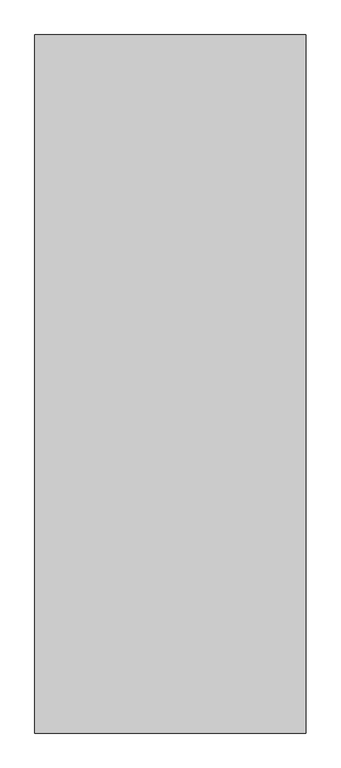
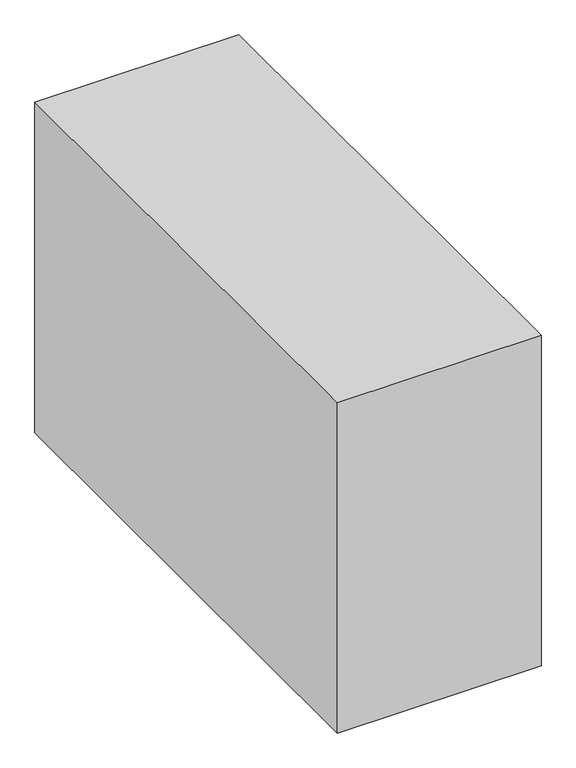
"""IFC4 building model written with IfcOpenShell, lengths in millimetres: proxy geometry, Space Planning Box_hec : Space Planning Box_hec."""

from ifc_helpers import new_model, si_unit, origin, origin_with_axes, place, context, project, spatial, polyline, outline, extrude, source, transform, mapped, element, save


def generic_models_c01b8d6f(model_context):
    return source(origin(), model_context, "Body", "SweptSolid", [
        extrude(outline(polyline([(1750.0, 4500.0), (1750.0, -4500.0), (-1750.0, -4500.0), (-1750.0, 4500.0), (1750.0, 4500.0)])), origin_with_axes(), (0.0, 0.0, 1.0), 6000.0),
    ])


if __name__ == "__main__":
    model = new_model("IFC4")
    model_context = context("Model", 3, world=origin())
    ifc_project = project(units=[si_unit("LENGTHUNIT", "METRE", prefix="MILLI")], contexts=[model_context])
    site = spatial("IfcSite", under=ifc_project)
    building = spatial("IfcBuilding", under=site)
    placement = place(None, origin())
    generic_models_shape = generic_models_c01b8d6f(model_context)
    element("IfcBuildingElementProxy", 1, Name="Space Planning Box_hec : Space Planning Box_hec", ObjectType="Space Planning Box_hec : Space Planning Box_hec", at=placement, inside=building, context=model_context, shape_type="MappedRepresentation", body=[
        mapped(generic_models_shape, transform((0.0, 0.0, 0.0), x_axis=(1.0, 0.0, 0.0), y_axis=(0.0, 1.0, 0.0), z_axis=(0.0, 0.0, 1.0))),
    ])
    save(model, "model.ifc")

# Revit data of these elements
# Type "Space Planning Box_hec : Space Planning Box_hec"
#   Type Comments = "..."
#   Room Name [instance default] = "?"
#   Interior Finish [instance default] = ""
#   Exterior Finish [instance default] = ""
#   Department [instance default] = ""
#   Assembly Code = "..."
#   Width [instance default] = 1524 mm
#   Program Area [instance default] = 0.00 m²
#   Length [instance default] = 1524 mm
#   Height [instance default] = 1524 mm
#   Area [instance default] = 2.32258 m²
#   Fill Color [instance default] = Cyan
#   Default Elevation = 0
# Element 1 (IfcBuildingElementProxy, "Space Planning Box_hec : Space Planning Box_hec")
#   Room Name = "Kitch & Lunch Room"
#   Interior Finish = "IF2-1"
#   Exterior Finish = "EF1"
#   Department = "AR"
#   Width = 3500 mm
#   Program Area = 31.50 m²
#   Length = 9000 mm
#   Height = 6000 mm
#   Area = 31.50 m²
#   Fill Color = Lavender
#   Materials on its faces: "Lavender"
# Materials
#   "Cyan": class "Generic", colour RGB 0 255 255, transparency 0.2, Cost = 0
#   "Lavender": class "Generic", colour RGB 186 85 211, transparency 0.2, Cost = 0
